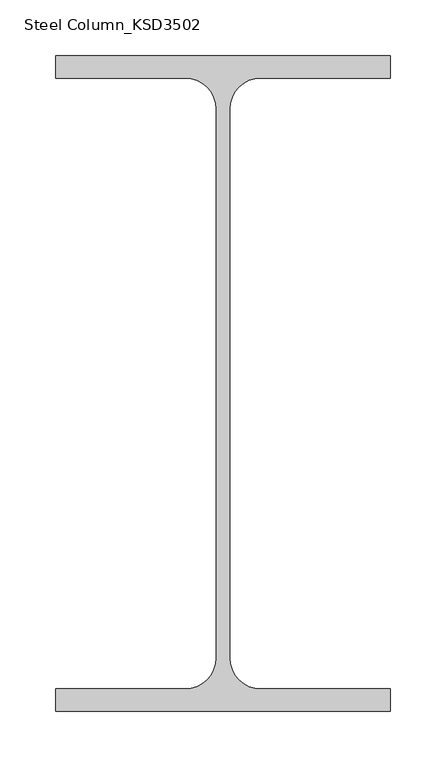
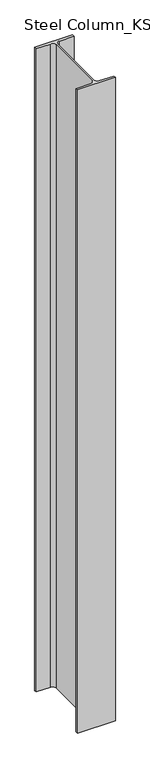
"""IFC4 building model written with IfcOpenShell, lengths in millimetres: column geometry, Steel Column_KSD3502 : H_SC_ASC_H-588×300x12x20."""

from ifc_helpers import new_model, si_unit, point, frame, frame_2d, origin, place, context, project, spatial, polyline, circle_curve, trimmed, segment, composite_curve, outline, extrude, source, transform, mapped, element, save


def steel_column_ksd3502_190025ee(model_context):
    return source(origin(), model_context, "Body", "SweptSolid", [
        extrude(outline(composite_curve([segment(polyline([(150.0, 294.0), (150.0, 274.0), (34.0, 274.0)]), True, "CONTINUOUS"), segment(trimmed(circle_curve(frame_2d((34.0, 246.0)), 28.0), [point((34.0, 274.0))], [point((6.0, 246.0))], True, "CARTESIAN"), True, "CONTINUOUS"), segment(polyline([(6.0, 246.0), (6.0, -246.0)]), True, "CONTINUOUS"), segment(trimmed(circle_curve(frame_2d((34.0, -246.0)), 28.0), [point((6.0, -246.0))], [point((34.0, -274.0))], True, "CARTESIAN"), True, "CONTINUOUS"), segment(polyline([(34.0, -274.0), (150.0, -274.0), (150.0, -294.0), (-150.0, -294.0), (-150.0, -274.0), (-34.0, -274.0)]), True, "CONTINUOUS"), segment(trimmed(circle_curve(frame_2d((-34.0, -246.0)), 28.0), [point((-34.0, -274.0))], [point((-6.0, -246.0))], True, "CARTESIAN"), True, "CONTINUOUS"), segment(polyline([(-6.0, -246.0), (-6.0, 246.0)]), True, "CONTINUOUS"), segment(trimmed(circle_curve(frame_2d((-34.0, 246.0)), 28.0), [point((-6.0, 246.0))], [point((-34.0, 274.0))], True, "CARTESIAN"), True, "CONTINUOUS"), segment(polyline([(-34.0, 274.0), (-150.0, 274.0), (-150.0, 294.0), (150.0, 294.0)]), True, "CONTINUOUS")], self_intersect=False)), frame((0.0, 0.0, 11909.9720055), z_axis=(0.0, 0.0, 1.0), x_axis=(1.0, 0.0, 0.0)), (0.0, 0.0, 1.0), 5390.0),
    ])


if __name__ == "__main__":
    model = new_model("IFC4")
    model_context = context("Model", 3, world=origin())
    ifc_project = project(units=[si_unit("LENGTHUNIT", "METRE", prefix="MILLI")], contexts=[model_context])
    site = spatial("IfcSite", under=ifc_project)
    building = spatial("IfcBuilding", under=site)
    placement = place(None, origin())
    steel_column_ksd3502_shape = steel_column_ksd3502_190025ee(model_context)
    element("IfcColumn", 1, ObjectType="Steel Column_KSD3502 : H_SC_ASC_H-588×300x12x20", at=placement, inside=building, context=model_context, shape_type="MappedRepresentation", body=[
        mapped(steel_column_ksd3502_shape, transform((0.0, 0.0, 0.0), x_axis=(1.0, 0.0, 0.0), y_axis=(0.0, 1.0, 0.0), z_axis=(0.0, 0.0, 1.0))),
    ])
    save(model, "model.ifc")

# Revit data of these elements
# Type "Steel Column_KSD3502 : H_SC_ASC_H-588×300x12x20"
#   Width = 30.0 cm
#   Web Thickness = 1.2 cm
#   Web Fillet = 2.8 cm
#   Warping Constant = 7259040.0 cm⁶
#   Torsional Moment of Inertia = 192.717 cm⁴
#   Section Area = 192.5 cm²
#   Plastic Modulus weak axis = 928.0 cm³
#   Plastic Modulus strong axis = 4490.0 cm³
#   Perimeter = 1.27 m²/m
#   Nominal Weight = 151.00 kgf/m
#   Moment of Inertia weak axis = 9020.00 cm⁴
#   Moment of Inertia strong axis = 118000.00 cm⁴
#   Height = 58.8 cm
#   Flange Thickness = 2.0 cm
#   Elastic Modulus weak axis = 601.0 cm³
#   Elastic Modulus strong axis = 4020.0 cm³
#   Centroid Vertical = 29.4 cm
#   Centroid Horizontal = 15.0 cm
#   Bolt Spacing = 13.97 cm
#   Structural Material [instance default] = Steel, 45-345
#   Section Name Key = ""
#   Assembly Code = ""
# Element 1 (IfcColumn, "Steel Column_KSD3502 : H_SC_ASC_H-588×300x12x20")
#   Structural Material = none
# Materials
#   "Steel, 45-345": class "Metal", colour RGB 189 187 185, transparency 0, Description = "Steel 345 MPa", Cost = 0
